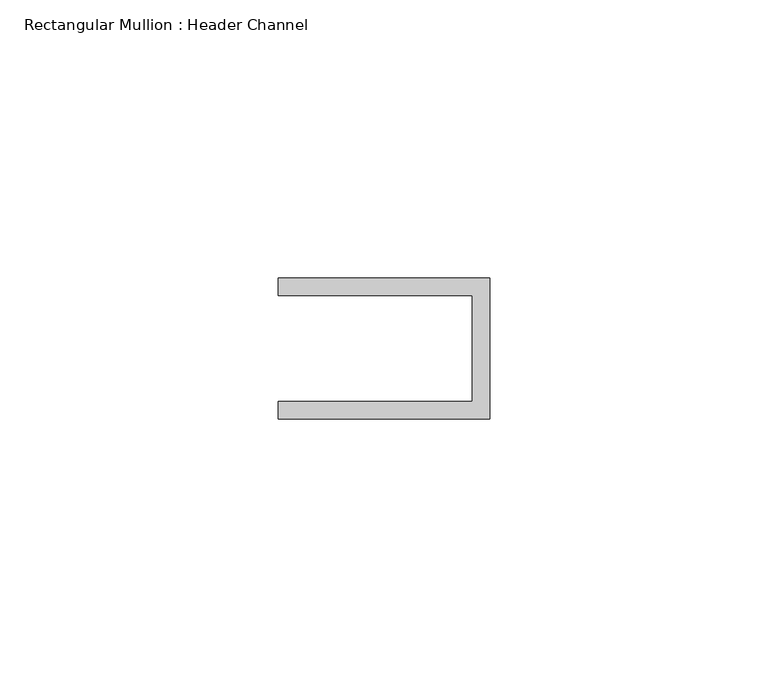
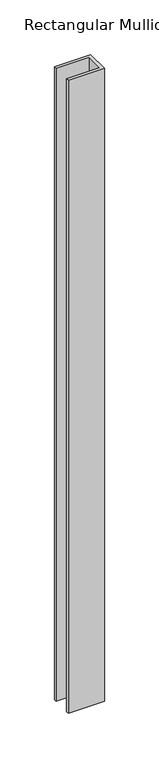
"""IFC4 building model written with IfcOpenShell, lengths in millimetres: member geometry, Rectangular Mullion : Header Channel."""

from ifc_helpers import new_model, si_unit, frame, origin, place, context, project, spatial, polyline, outline, extrude, source, transform, mapped, element, save


def rectangular_mullion_header_channel_d9c98084(model_context):
    return source(origin(), model_context, "Body", "SweptSolid", [
        extrude(outline(polyline([(0.0, -12.7), (-38.1, -12.7), (-38.1, -9.525), (-3.175, -9.525), (-3.175, 9.525), (-38.1, 9.525), (-38.1, 12.7), (0.0, 12.7), (0.0, -12.7)])), frame((0.0, 0.0, -706.9666667), z_axis=(0.0, 0.0, 1.0), x_axis=(1.0, 0.0, 0.0)), (0.0, 0.0, 1.0), 706.9666667),
    ])


if __name__ == "__main__":
    model = new_model("IFC4")
    model_context = context("Model", 3, world=origin())
    ifc_project = project(units=[si_unit("LENGTHUNIT", "METRE", prefix="MILLI")], contexts=[model_context])
    site = spatial("IfcSite", under=ifc_project)
    building = spatial("IfcBuilding", under=site)
    placement = place(None, origin())
    rectangular_mullion_header_channel_shape = rectangular_mullion_header_channel_d9c98084(model_context)
    element("IfcMember", 1, ObjectType="Rectangular Mullion : Header Channel", at=placement, inside=building, context=model_context, shape_type="MappedRepresentation", body=[
        mapped(rectangular_mullion_header_channel_shape, transform((0.0, 0.0, 0.0), x_axis=(1.0, 0.0, 0.0), y_axis=(0.0, 1.0, 0.0), z_axis=(0.0, 0.0, 1.0))),
    ])
    save(model, "model.ifc")

# Revit data of these elements
# Type "Rectangular Mullion : Header Channel"
#   built-in parameter 1007322 = 0.0833333 (stored number, unit not read)
#   built-in parameter 1007321 = -0.03125 (stored number, unit not read)
#   built-in parameter 1007320 = 0.0416667 (stored number, unit not read)
# Element 1 (IfcMember, "Rectangular Mullion : Header Channel")
#   Materials on its faces: "ALUM"
# Materials
#   "ALUM": class "Generic", colour RGB 157 157 157, transparency 0, Cost = 0
